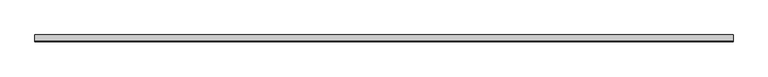
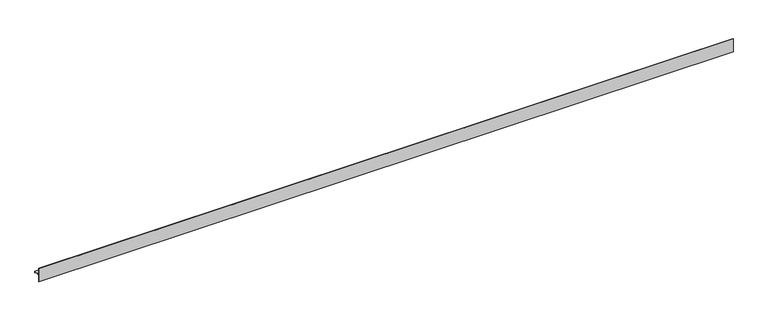
"""IFC4 building model written with IfcOpenShell, lengths in millimetres: proxy geometry, Metal profile003 534 : Metal profile003 534."""

from ifc_helpers import new_model, si_unit, frame, origin, place, context, project, spatial, polyline, outline, extrude, source, transform, mapped, element, save


def generic_models_84f21a9e(model_context):
    return source(origin(), model_context, "Body", "SweptSolid", [
        extrude(outline(polyline([(9773.5175834, 37481.0682813), (9756.5536354, 37481.0682813), (9756.5536354, 37462.0182812), (9755.2836354, 37462.0182812), (9755.2836354, 37501.3882813), (9756.5536354, 37501.3882813), (9756.5536354, 37482.3382813), (9774.7875834, 37482.3382813), (9774.7875834, 37477.5884813), (9773.5175834, 37477.5884813), (9773.5175834, 37481.0682813)])), frame((3694.2883192, 0.0, 0.0), z_axis=(1.0, 0.0, 0.0), x_axis=(0.0, 1.0, 0.0)), (0.0, 0.0, 1.0), 2000.0),
    ])


if __name__ == "__main__":
    model = new_model("IFC4")
    model_context = context("Model", 3, world=origin())
    ifc_project = project(units=[si_unit("LENGTHUNIT", "METRE", prefix="MILLI")], contexts=[model_context])
    site = spatial("IfcSite", under=ifc_project)
    building = spatial("IfcBuilding", under=site)
    placement = place(None, origin())
    generic_models_shape = generic_models_84f21a9e(model_context)
    element("IfcBuildingElementProxy", 1, Name="Metal profile003 534 : Metal profile003 534", ObjectType="Metal profile003 534 : Metal profile003 534", at=placement, inside=building, context=model_context, shape_type="MappedRepresentation", body=[
        mapped(generic_models_shape, transform((0.0, 0.0, 0.0), x_axis=(1.0, 0.0, 0.0), y_axis=(0.0, 1.0, 0.0), z_axis=(0.0, 0.0, 1.0))),
    ])
    save(model, "model.ifc")

# Revit data of these elements
# Type "Metal profile003 534 : Metal profile003 534"
#   NameOverride = "Metal profile003"
# Element 1 (IfcBuildingElementProxy, "Metal profile003 534 : Metal profile003 534")
#   Materials on its faces: "16 GA. COPPER VENTED T REVEAL BEAD"
# Materials
#   "16 GA. COPPER VENTED T REVEAL BEAD": class "Unassigned", colour RGB 255 227 10, transparency 0
